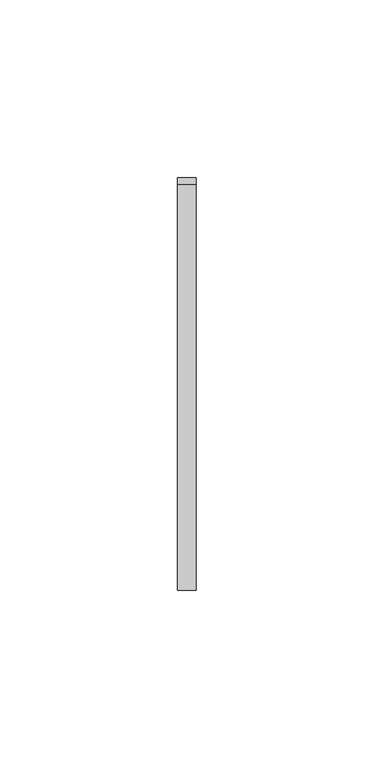
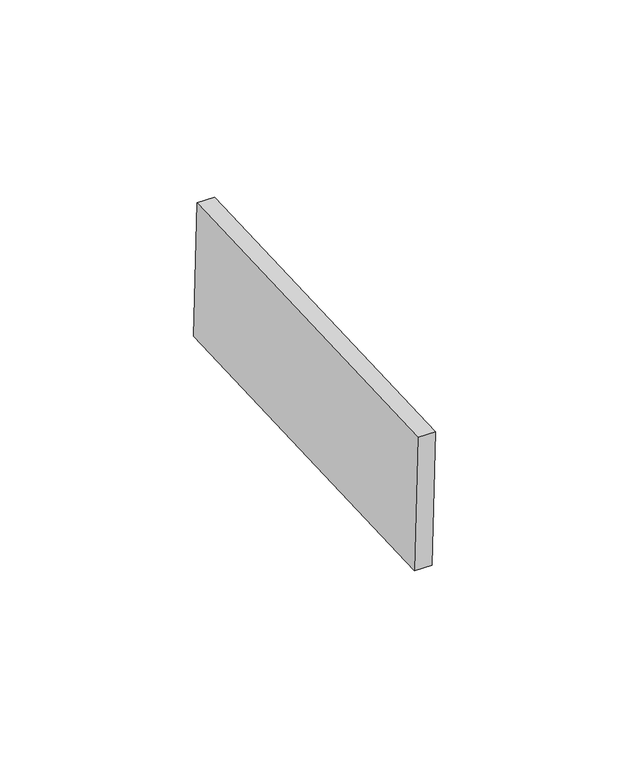
"""IFC4 building model written with IfcOpenShell, lengths in millimetres: proxy geometry, Inner panel:Inner panel:1:Inner panel:1 : Inner panel:Inner panel:300324:2:Inner panel:1:Inner panel:1 : Inner panel:Inner panel:300324:2 : Inner panel:Inner panel:1:Inner panel:1 : Inner panel:Inner panel:300324:300043:78 : Inner panel:Inner panel:1:Inner panel:1 : Inner panel:Inner panel:300324:2:Inner panel:1:Inner panel:1 : Inner panel:Inner panel:300324:2 : Inner panel:Inner panel:1:Inner panel:1 : Inner panel:Inner panel:300324:300043:308120."""

from ifc_helpers import new_model, si_unit, frame, origin, place, context, project, spatial, polyline, outline, extrude, source, transform, mapped, element, save


def generic_models_b7f0b5dc(model_context):
    return source(origin(), model_context, "Body", "SweptSolid", [
        extrude(outline(polyline([(0.0, -114.3), (0.0, 0.0), (5.2138089, 0.0), (5.2138089, -114.3), (0.0, -114.3)])), frame((592310.995117, -578297.797364, 3981.6641254), z_axis=(0.0, -0.04163054471216399, 0.9991330730923527), x_axis=(-1.0, 0.0, 0.0)), (0.0, 0.0, 1.0), 43.2233908),
    ])


if __name__ == "__main__":
    model = new_model("IFC4")
    model_context = context("Model", 3, world=origin())
    ifc_project = project(units=[si_unit("LENGTHUNIT", "METRE", prefix="MILLI")], contexts=[model_context])
    site = spatial("IfcSite", under=ifc_project)
    building = spatial("IfcBuilding", under=site)
    placement = place(None, origin())
    generic_models_shape = generic_models_b7f0b5dc(model_context)
    element("IfcBuildingElementProxy", 1, Name="Inner panel:Inner panel:1:Inner panel:1 : Inner panel:Inner panel:300324:2:Inner panel:1:Inner panel:1 : Inner panel:Inner panel:300324:2 : Inner panel:Inner panel:1:Inner panel:1 : Inner panel:Inner panel:300324:300043:78 : Inner panel:Inner panel:1:Inner panel:1 : Inner panel:Inner panel:300324:2:Inner panel:1:Inner panel:1 : Inner panel:Inner panel:300324:2 : Inner panel:Inner panel:1:Inner panel:1 : Inner panel:Inner panel:300324:300043:308120", ObjectType="Inner panel:Inner panel:1:Inner panel:1 : Inner panel:Inner panel:300324:2:Inner panel:1:Inner panel:1 : Inner panel:Inner panel:300324:2 : Inner panel:Inner panel:1:Inner panel:1 : Inner panel:Inner panel:300324:300043:78 : Inner panel:Inner panel:1:Inner panel:1 : Inner panel:Inner panel:300324:2:Inner panel:1:Inner panel:1 : Inner panel:Inner panel:300324:2 : Inner panel:Inner panel:1:Inner panel:1 : Inner panel:Inner panel:300324:300043:308120", at=placement, inside=building, context=model_context, shape_type="MappedRepresentation", body=[
        mapped(generic_models_shape, transform((0.0, 0.0, 0.0), x_axis=(1.0, 0.0, 0.0), y_axis=(0.0, 1.0, 0.0), z_axis=(0.0, 0.0, 1.0))),
    ])
    save(model, "model.ifc")

# Revit data of these elements
# Type "Inner panel:Inner panel:1:Inner panel:1 : Inner panel:Inner panel:300324:2:Inner panel:1:Inner panel:1 : Inner panel:Inner panel:300324:2 : Inner panel:Inner panel:1:Inner panel:1 : Inner panel:Inner panel:300324:300043:78 : Inner panel:Inner panel:1:Inner panel:1 : Inner panel:Inner panel:300324:2:Inner panel:1:Inner panel:1 : Inner panel:Inner panel:300324:2 : Inner panel:Inner panel:1:Inner panel:1 : Inner panel:Inner panel:300324:300043:308120"
#   NameOverride = "Inner panel:Inner panel:1:Inner panel:1 : Inner panel:Inner panel:300324:2:Inner panel:1:Inner panel:1 : Inner panel:Inner panel:300324:2 : Inner panel:Inner panel:1:Inner panel:1 : Inner panel:Inner panel:300324:300043:308120"
#   ObjectTypeOverride = "Inner panel:1:Inner panel:1 : Inner panel:Inner panel:300324:2 : Inner panel:Inner panel:1:Inner panel:1 : Inner panel:Inner panel:300324:300043"
#   Reference = "Inner panel"
#   Tag = "308120"
# Element 1 (IfcBuildingElementProxy, "Inner panel:Inner panel:1:Inner panel:1 : Inner panel:Inner panel:300324:2:Inner panel:1:Inner panel:1 : Inner panel:Inner panel:300324:2 : Inner panel:Inner panel:1:Inner panel:1 : Inner panel:Inner panel:300324:300043:78 : Inner panel:Inner panel:1:Inner panel:1 : Inner panel:Inner panel:300324:2:Inner panel:1:Inner panel:1 : Inner panel:Inner panel:300324:2 : Inner panel:Inner panel:1:Inner panel:1 : Inner panel:Inner panel:300324:300043:308120")
#   Materials on its faces: "SLIDING CLIP"
# Materials
#   "SLIDING CLIP": class "Generic", colour RGB 120 120 120, transparency 0, Cost = 0
